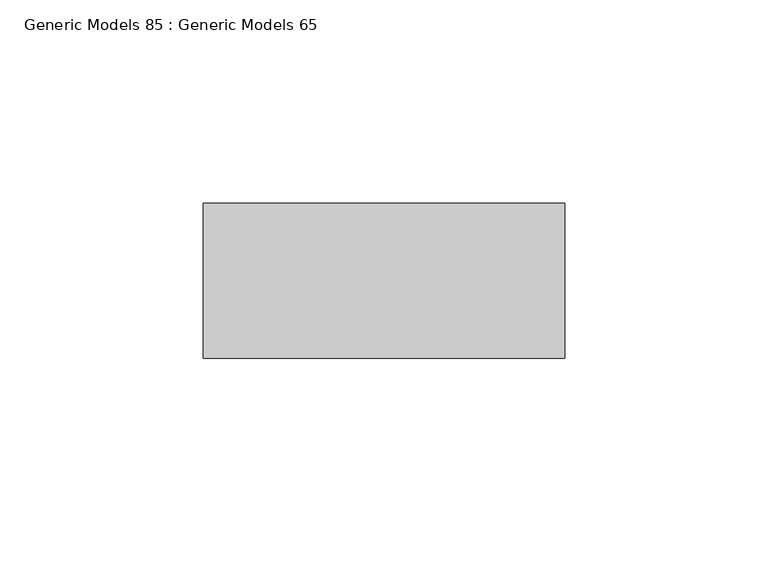
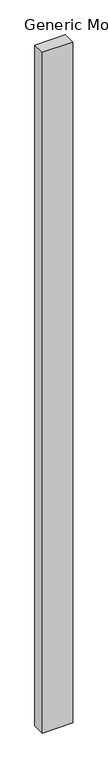
"""IFC4 building model written with IfcOpenShell, lengths in millimetres: proxy geometry, Generic Models 85 : Generic Models 65."""

from ifc_helpers import new_model, si_unit, frame, origin, place, context, project, spatial, polyline, outline, extrude, source, transform, mapped, element, save


def generic_models_85_generic_models_65_bcc3fffd(model_context):
    return source(origin(), model_context, "Body", "SweptSolid", [
        extrude(outline(polyline([(52222.4, 592.1375), (52133.5, 592.1375), (52133.5, 630.2375), (52222.4, 630.2375), (52222.4, 592.1375)])), frame((0.0, 0.0, 3086.1), z_axis=(0.0, 0.0, 1.0), x_axis=(1.0, 0.0, 0.0)), (0.0, 0.0, 1.0), 2098.278125),
    ])


if __name__ == "__main__":
    model = new_model("IFC4")
    model_context = context("Model", 3, world=origin())
    ifc_project = project(units=[si_unit("LENGTHUNIT", "METRE", prefix="MILLI")], contexts=[model_context])
    site = spatial("IfcSite", under=ifc_project)
    building = spatial("IfcBuilding", under=site)
    placement = place(None, origin())
    generic_models_85_generic_models_65_shape = generic_models_85_generic_models_65_bcc3fffd(model_context)
    element("IfcBuildingElementProxy", 1, Name="Generic Models 85 : Generic Models 65", ObjectType="Generic Models 85 : Generic Models 65", at=placement, inside=building, context=model_context, shape_type="MappedRepresentation", body=[
        mapped(generic_models_85_generic_models_65_shape, transform((0.0, 0.0, 0.0), x_axis=(1.0, 0.0, 0.0), y_axis=(0.0, 1.0, 0.0), z_axis=(0.0, 0.0, 1.0))),
    ])
    save(model, "model.ifc")

# Revit data of these elements
# Element 1 (IfcBuildingElementProxy, "Generic Models 85 : Generic Models 65")
#   Materials on its faces: "2X WOOD STUD - SEE 'WALL TAG' & 'LAYER MATERIAL SCHEDULE' FOR SPACING & INSULATION TREATMENT, IF APPLICAPLE"
# Materials
#   "2X WOOD STUD - SEE 'WALL TAG' & 'LAYER MATERIAL SCHEDULE' FOR SPACING & INSULATION TREATMENT, IF APPLICAPLE": class "Wood", colour RGB 234 198 147, transparency 0, Description = "Pinus Echinata", Cost = 0
